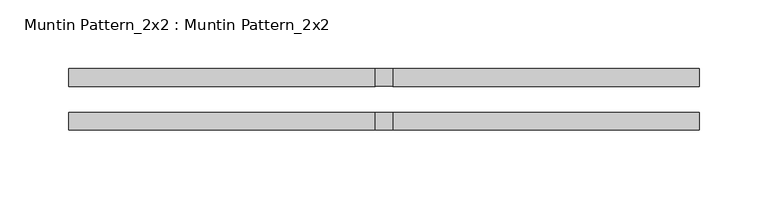
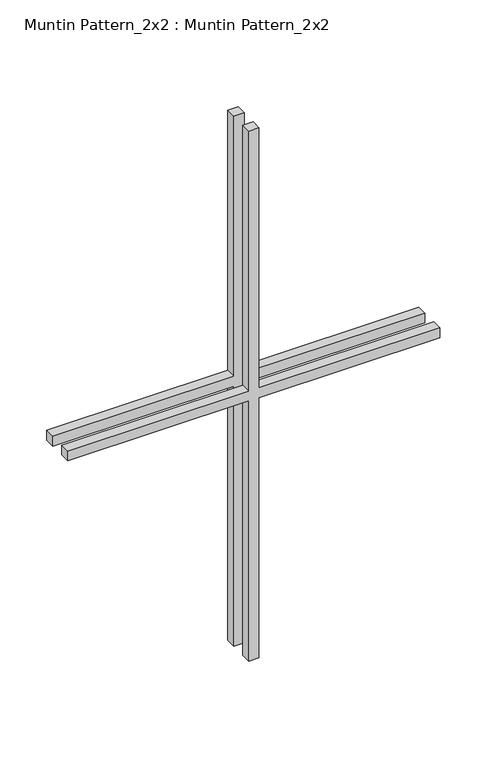
"""IFC4 building model written with IfcOpenShell, lengths in millimetres: proxy geometry, Muntin Pattern_2x2 : Muntin Pattern_2x2."""

from ifc_helpers import new_model, si_unit, frame, origin, place, context, project, spatial, polyline, outline, extrude, source, transform, mapped, element, save


def muntin_pattern_2x2_muntin_pattern_2x2_d7e7d62e(model_context):
    return source(origin(), model_context, "Body", "SweptSolid", [
        extrude(outline(polyline([(350.8375, -6.35), (350.8375, -228.6), (338.1375, -228.6), (338.1375, -6.35), (0.0, -6.35), (0.0, 6.35), (338.1375, 6.35), (338.1375, 228.6), (350.8375, 228.6), (350.8375, 6.35), (688.975, 6.35), (688.975, -6.35), (350.8375, -6.35)])), frame((0.0, 9.525, 0.0), z_axis=(0.0, 1.0, 0.0), x_axis=(0.0, 0.0, 1.0)), (0.0, 0.0, 1.0), 12.7),
        extrude(outline(polyline([(350.8375, -6.35), (350.8375, -228.6), (338.1375, -228.6), (338.1375, -6.35), (0.0, -6.35), (0.0, 6.35), (338.1375, 6.35), (338.1375, 228.6), (350.8375, 228.6), (350.8375, 6.35), (688.975, 6.35), (688.975, -6.35), (350.8375, -6.35)])), frame((0.0, -22.225, 0.0), z_axis=(0.0, 1.0, 0.0), x_axis=(0.0, 0.0, 1.0)), (0.0, 0.0, 1.0), 12.7),
    ])


if __name__ == "__main__":
    model = new_model("IFC4")
    model_context = context("Model", 3, world=origin())
    ifc_project = project(units=[si_unit("LENGTHUNIT", "METRE", prefix="MILLI")], contexts=[model_context])
    site = spatial("IfcSite", under=ifc_project)
    building = spatial("IfcBuilding", under=site)
    placement = place(None, origin())
    muntin_pattern_2x2_muntin_pattern_2x2_shape = muntin_pattern_2x2_muntin_pattern_2x2_d7e7d62e(model_context)
    element("IfcBuildingElementProxy", 1, Name="Muntin Pattern_2x2 : Muntin Pattern_2x2", ObjectType="Muntin Pattern_2x2 : Muntin Pattern_2x2", at=placement, inside=building, context=model_context, shape_type="MappedRepresentation", body=[
        mapped(muntin_pattern_2x2_muntin_pattern_2x2_shape, transform((0.0, 0.0, 0.0), x_axis=(1.0, 0.0, 0.0), y_axis=(0.0, 1.0, 0.0), z_axis=(0.0, 0.0, 1.0))),
    ])
    save(model, "model.ifc")

# Revit data of these elements
# Type "Muntin Pattern_2x2 : Muntin Pattern_2x2"
#   Width [instance default] = 4' - 0"
#   Thickness = 0' - 0 1/2"
#   Height [instance default] = 4' - 0"
#   Distance = 0' - 0 3/4"
#   Interior Material [instance default] = none
#   Exterior Material [instance default] = none
#   Default Elevation = 0
# Element 1 (IfcBuildingElementProxy, "Muntin Pattern_2x2 : Muntin Pattern_2x2")
#   Width = 1' - 6"
#   Height = 2' - 3 1/8"
#   Interior Material = Wood - Stained
#   Exterior Material = Clad - White
#   Materials on its faces: "Clad - White", "Wood - Stained"
# Materials
#   "Clad - White": class "Wood", colour RGB 245 245 243, transparency 0, Cost = 0
#   "Wood - Stained": class "Wood", colour RGB 224 178 126, transparency 0, Cost = 0
